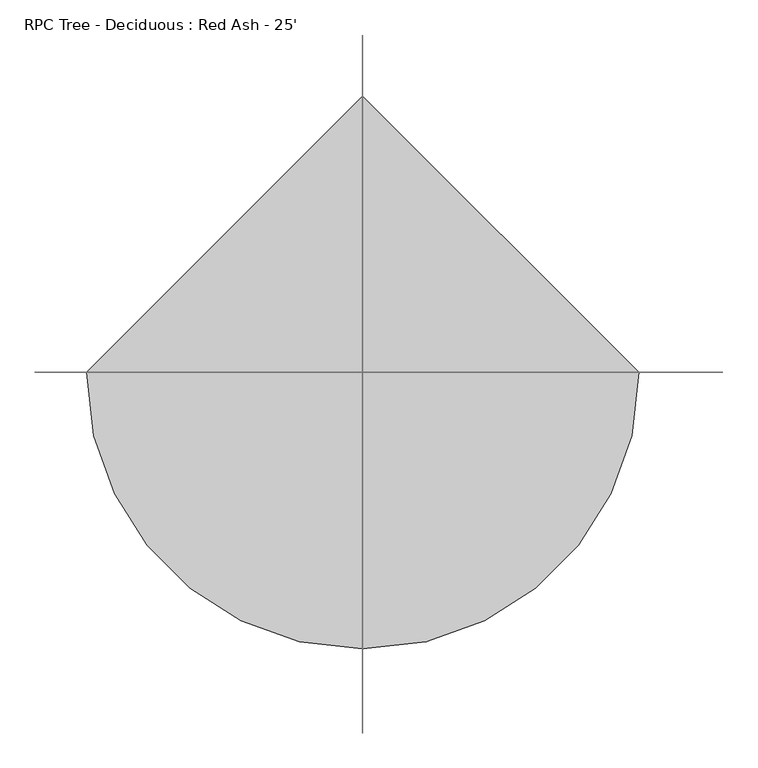
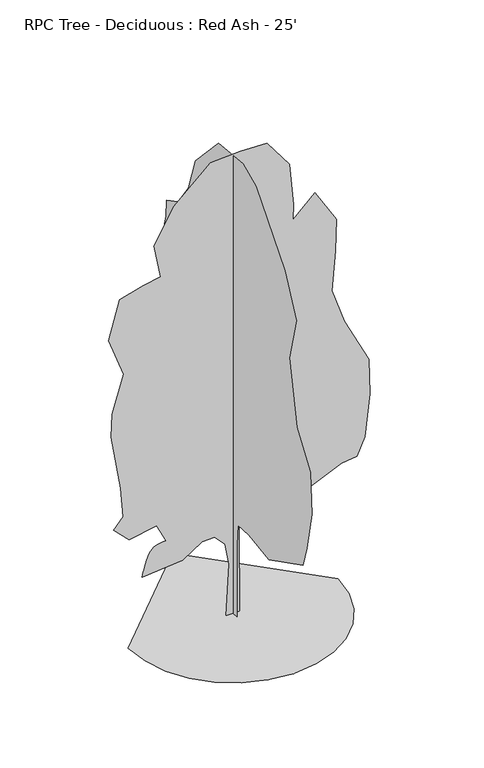
"""IFC4 building model written with IfcOpenShell, lengths in millimetres: geographic element geometry, RPC Tree - Deciduous : Red Ash - 25'."""

import ifcopenshell
import ifcopenshell.guid

model = None  # the IFC model being written
_history = None  # IfcOwnerHistory: only IFC2X3 demands one
_inside = {}  # id of a spatial element -> (the spatial element, [elements in it])
_under = {}  # id of a project, library or spatial element -> (it, [spatial elements below it])
_declared = {}  # id of a project -> (the project, [libraries it declares])
_typed = {}  # id of a type object -> (the type object, [elements of that type])
_made_of = {}  # id of a material, layer set ... -> (it, [elements and type objects made of it])


def new_model(schema):
    """Start an empty IFC model of exactly this schema.

    Asked for "IFC4X3", IfcOpenShell would pick the latest addendum, in which some entities
    have other attributes; the version numbers below select the first issue.
    IFC2X3 requires an IfcOwnerHistory on every rooted entity: one is made here for all.
    """
    global model, _history
    if schema == "IFC4X3":
        model = ifcopenshell.file(schema_version=(4, 3, 0, 0))
    else:
        model = ifcopenshell.file(schema=schema)
    _inside.clear()
    _under.clear()
    _declared.clear()
    _typed.clear()
    _made_of.clear()
    _history = None
    if model.schema == "IFC2X3":
        org = make("IfcOrganization", Name="unknown")
        user = make(
            "IfcPersonAndOrganization",
            ThePerson=make("IfcPerson", FamilyName="unknown"),
            TheOrganization=org,
        )
        app = make(
            "IfcApplication",
            ApplicationDeveloper=org,
            Version="unknown",
            ApplicationFullName="unknown",
            ApplicationIdentifier="unknown",
        )
        _history = make(
            "IfcOwnerHistory",
            OwningUser=user,
            OwningApplication=app,
            ChangeAction="ADDED",
            CreationDate=0,
        )
    return model


def make(cls, **values):
    """One entity of the class cls with the attributes given. An attribute that is None is left unset."""
    return model.create_entity(
        cls, **{name: value for name, value in values.items() if value is not None}
    )


def rooted(cls, **values):
    """An entity with a GlobalId (a new one), such as an element, a storey or a relation."""
    return make(cls, GlobalId=ifcopenshell.guid.new(), OwnerHistory=_history, **values)


def si_unit(unit_type, name, prefix=None):
    """IfcSIUnit, for example si_unit("LENGTHUNIT", "METRE", prefix="MILLI")."""
    return make("IfcSIUnit", UnitType=unit_type, Prefix=prefix, Name=name)


def assignment(units):
    """IfcUnitAssignment: the units of a project."""
    return None if units is None else make("IfcUnitAssignment", Units=units)


def point(xyz):
    """IfcCartesianPoint."""
    return None if xyz is None else make("IfcCartesianPoint", Coordinates=xyz)


def direction(xyz):
    """IfcDirection."""
    return None if xyz is None else make("IfcDirection", DirectionRatios=xyz)


def frame(location, z_axis=None, x_axis=None):
    """IfcAxis2Placement3D, a coordinate frame: its origin and axes. An axis left out is left unset."""
    return make(
        "IfcAxis2Placement3D",
        Location=point(location),
        Axis=direction(z_axis),
        RefDirection=direction(x_axis),
    )


def origin():
    """The frame at (0, 0, 0) with its axes left unset."""
    return frame((0.0, 0.0, 0.0))


def place(relative_to, where):
    """IfcLocalPlacement: puts the frame where relative to a parent placement (None: the world)."""
    return make(
        "IfcLocalPlacement", PlacementRelTo=relative_to, RelativePlacement=where
    )


def context(
    kind, dimensions, precision=None, world=None, true_north=None, identifier=None
):
    """IfcGeometricRepresentationContext, for example the 3D "Model" context."""
    return make(
        "IfcGeometricRepresentationContext",
        ContextIdentifier=identifier,
        ContextType=kind,
        CoordinateSpaceDimension=dimensions,
        Precision=precision,
        WorldCoordinateSystem=world,
        TrueNorth=true_north,
    )


def project(units=None, contexts=None):
    """IfcProject with its units and contexts."""
    return rooted(
        "IfcProject",
        Name="project",
        RepresentationContexts=contexts,
        UnitsInContext=assignment(units),
    )


def spatial(cls, under=None, at=None, **own):
    """A site, building, storey or space (cls), placed at a placement, below another one or the project."""
    s = rooted(cls, ObjectPlacement=at, **own)
    if under is not None:
        _under.setdefault(under.id(), (under, []))[1].append(s)
    return s


def point_list(points):
    """IfcCartesianPointList2D or 3D."""
    cls = (
        "IfcCartesianPointList2D" if len(points[0]) == 2 else "IfcCartesianPointList3D"
    )
    return make(cls, CoordList=points)


def triangles(points, corners, closed=None, point_numbers=None):
    """IfcTriangulatedFaceSet: each triangle names its three corners, points numbered from 1."""
    return make(
        "IfcTriangulatedFaceSet",
        Coordinates=point_list(points),
        Closed=closed,
        CoordIndex=corners,
        PnIndex=point_numbers,
    )


def shape(context_of_items, identifier, shape_type, items):
    """IfcShapeRepresentation: the items that make up one representation, for example the "Body"."""
    return make(
        "IfcShapeRepresentation",
        ContextOfItems=context_of_items,
        RepresentationIdentifier=identifier,
        RepresentationType=shape_type,
        Items=items,
    )


def source(mapping_origin, context_of_items, identifier, shape_type, items):
    """IfcRepresentationMap: a shape defined once, which mapped items show again and again."""
    return make(
        "IfcRepresentationMap",
        MappingOrigin=mapping_origin,
        MappedRepresentation=shape(context_of_items, identifier, shape_type, items),
    )


def transform(
    local_origin,
    x_axis=None,
    y_axis=None,
    z_axis=None,
    scale=None,
    scale2=None,
    scale3=None,
    uniform=True,
):
    """IfcCartesianTransformationOperator3D, or its non-uniform kind. x_axis, y_axis, z_axis: its Axis1, 2, 3."""
    if uniform:
        return make(
            "IfcCartesianTransformationOperator3D",
            Axis1=direction(x_axis),
            Axis2=direction(y_axis),
            LocalOrigin=point(local_origin),
            Scale=scale,
            Axis3=direction(z_axis),
        )
    return make(
        "IfcCartesianTransformationOperator3DnonUniform",
        Axis1=direction(x_axis),
        Axis2=direction(y_axis),
        LocalOrigin=point(local_origin),
        Scale=scale,
        Axis3=direction(z_axis),
        Scale2=scale2,
        Scale3=scale3,
    )


def mapped(mapping_source, mapping_target):
    """IfcMappedItem: shows the shape of a source again, moved by a transform."""
    return make(
        "IfcMappedItem", MappingSource=mapping_source, MappingTarget=mapping_target
    )


def made_of(thing, what):
    """Note that an element or type object is made of a material, layer set ...; save() writes the relation."""
    if what is not None:
        _made_of.setdefault(what.id(), (what, []))[1].append(thing)
    return thing


def element(
    cls,
    number,
    at=None,
    inside=None,
    cuts=None,
    type_object=None,
    material=None,
    context=None,
    identifier="Body",
    shape_type=None,
    held_by="IfcProductDefinitionShape",
    body=None,
    shapes=None,
    **own,
):
    """One element of the class cls, such as IfcWall. Its Tag is "e" and its number.

    at: its placement. inside: the storey or other place that contains it. cuts: it is an
    opening in that element (IfcRelVoidsElement). A single representation is given by context,
    identifier, shape_type and body (its items); several are given by shapes. held_by: the class
    of the entity that holds the representations. save() writes the other relations.
    """
    e = rooted(cls, Tag="e%d" % number, ObjectPlacement=at, **own)
    if body is not None:
        shapes = [shape(context, identifier, shape_type, body)]
    if shapes is not None:
        e.Representation = make(held_by, Representations=shapes)
    if inside is not None:
        _inside.setdefault(inside.id(), (inside, []))[1].append(e)
    if cuts is not None:
        rooted(
            "IfcRelVoidsElement", RelatingBuildingElement=cuts, RelatedOpeningElement=e
        )
    if type_object is not None:
        _typed.setdefault(type_object.id(), (type_object, []))[1].append(e)
    return made_of(e, material)


def aggregate(whole, parts):
    """IfcRelAggregates: a whole, such as a stair, and the parts it consists of."""
    return rooted("IfcRelAggregates", RelatingObject=whole, RelatedObjects=parts)


def save(model, path):
    """Write the relations noted so far, then the file.

    IfcRelAggregates (storeys below a building ...), IfcRelContainedInSpatialStructure (elements
    in a storey), IfcRelDefinesByType, IfcRelAssociatesMaterial and IfcRelDeclares: one each for
    every whole, place, type object, material and project.
    """
    for whole, parts in _under.values():
        aggregate(whole, parts)
    for where, things in _inside.values():
        rooted(
            "IfcRelContainedInSpatialStructure",
            RelatedElements=things,
            RelatingStructure=where,
        )
    for kind, things in _typed.values():
        rooted("IfcRelDefinesByType", RelatedObjects=things, RelatingType=kind)
    for what, things in _made_of.values():
        rooted("IfcRelAssociatesMaterial", RelatedObjects=things, RelatingMaterial=what)
    for by, libraries in _declared.values():
        rooted("IfcRelDeclares", RelatingContext=by, RelatedDefinitions=libraries)
    model.write(path)


def rpc_tree_deciduous_red_ash_25_14781bec(model_context):
    return source(origin(), model_context, "Body", "Tessellation", [
        triangles([(-1644.9525009, 0.0, 6.19e-05), (-1601.4651844, -376.9143482, 6.19e-05), (-1477.6144592, -723.0498339, 6.19e-05), (-1283.3164352, -1028.4894024, 6.19e-05), (-1028.4894751, -1283.3165806, 6.19e-05), (-723.0496885, -1477.6140232, 6.19e-05), (-376.9141665, -1601.4651844, 6.19e-05), (7.19e-05, -1644.9525009, 6.19e-05), (376.9143846, -1601.4651844, 6.19e-05), (723.0499065, -1477.6143139, 6.19e-05), (1028.4894751, -1283.3164352, 6.19e-05), (1283.3168713, -1028.4894751, 6.19e-05), (1477.6141685, -723.0496159, 6.19e-05), (1601.4651844, -376.9140939, 6.19e-05), (1644.9525009, 0.0001438, 6.19e-05), (-0.0002157, 1644.9525009, 6.19e-05), (-1.07e-05, -102.8462569, 0.0), (2.5e-05, -101.2467179, 1194.554048), (3.23e-05, -129.8819613, 1537.8029366), (7e-07, -438.8253948, 1558.1655018), (-5.78e-05, -976.3912743, 1478.3068588), (-0.0001405, -1903.692667, 1948.6771305), (-0.0001413, -2011.2060173, 2298.095192), (-0.0001361, -2145.5975235, 2943.1744217), (-0.0001119, -2105.2803623, 3615.1319527), (-5.81e-05, -1740.3819958, 4141.0172951), (-5.5e-06, -1527.3986298, 5160.6350006), (-3.5e-06, -1715.5451397, 5886.3488434), (4.79e-05, -1406.4449661, 6531.4286545), (0.0001569, -626.9743755, 7458.7301926), (0.0001985, -273.2007115, 7618.1942963), (0.0002662, 394.4016166, 7552.8046829), (0.0003121, 1026.0418774, 6880.8468613), (0.0003149, 1214.190204, 6316.4022446), (0.0003323, 1496.411277, 5913.2274353), (0.0003598, 1805.5131947, 5751.9582092), (0.0003531, 1818.9521999, 5483.1746155), (0.0003523, 1899.587249, 5174.0742966), (0.0003275, 1765.1957428, 4811.2170845), (0.0003297, 1886.1480984, 4461.7991684), (0.0003279, 2007.1004539, 3977.9897461), (0.0003211, 1980.222298, 3843.5979492), (0.0002877, 1751.7567375, 3521.0580437), (0.0002729, 1737.3115437, 3077.5662186), (0.0002632, 1724.8782909, 2795.3439102), (0.0002542, 1738.3174416, 2445.9262848), (0.0002412, 1751.7568829, 1962.1167171), (0.0002172, 1563.6084835, 1814.2857697), (0.0001807, 1214.1907127, 1814.2857697), (0.0001827, 1375.4605202, 1317.0371967), (0.0001715, 1348.4951603, 1034.8845062), (0.0001516, 1103.0310734, 1227.8363914), (9.86e-05, 629.4626684, 1106.7075932), (9.8e-05, 551.7118183, 1357.0609165), (6.29e-05, 215.9127657, 1354.0025276), (5.03e-05, 130.8012366, 1228.3346169), (3.27e-05, 79.5493323, 818.2831198), (1.17e-05, 112.1660096, 1.28e-05), (-110.870867, 4.8e-06, 4.46e-05), (-66.7114758, -9.64e-05, 833.5016676), (-129.3072962, -0.000136, 1187.9435503), (-290.7878647, -0.00015, 1365.31768), (-483.6364677, -0.0001408, 1358.6964272), (-796.2678211, -0.000103, 1155.7673166), (-1427.9080456, -6.9e-05, 1102.0108595), (-1419.1706429, -7.35e-05, 1136.7646975), (-1409.8454853, -7.82e-05, 1172.6938271), (-1399.3449635, -8.32e-05, 1210.9736853), (-1387.0813225, -8.87e-05, 1252.7803631), (-1372.4668076, -9.49e-05, 1299.2876987), (-1354.9136639, -0.0001019, 1351.6733093), (-1333.8341366, -0.0001099, 1411.1111057), (-1307.2693336, -0.0001176, 1466.2392815), (-1274.3570984, -0.0001239, 1506.556588), (-1236.1555058, -0.0001289, 1534.5316246), (-1193.7220493, -0.0001329, 1552.6338627), (-1148.1152401, -0.0001362, 1563.3300121), (-1100.3923536, -0.000139, 1569.0895443), (-1051.6116829, -0.0001415, 1572.3809132), (-1199.4421944, -0.0001703, 1868.0423721), (-1629.4953049, -0.0001418, 1787.4073231), (-1871.3997253, -0.0001601, 2029.3124702), (-1723.5690685, -0.0001874, 2204.0214283), (-1763.886375, -0.0002433, 2687.8309959), (-1911.7170319, -0.0003442, 3588.2539421), (-1898.4807758, -0.0003892, 3961.1654823), (-1719.9175472, -0.0004688, 4563.3255295), (-1952.0346291, -0.0005347, 5200.9523071), (-1777.3253803, -0.000616, 5819.1535263), (-1414.4687496, -0.0006447, 5926.6667313), (-1138.413216, -0.0006626, 5975.3625961), (-1239.7599369, -0.0007228, 6517.9893585), (-930.6591093, -0.000802, 7068.9952606), (-352.7753057, -0.0008898, 7593.1219894), (117.5946844, -0.0009135, 7620.0), (534.2087442, -0.0009301, 7606.5601227), (883.626733, -0.0008893, 7136.1905777), (947.8720848, -0.00081, 6447.5180786), (938.6469212, -0.0007795, 6194.9695404), (1286.8011063, -0.0008333, 6517.9893585), (1622.7800171, -0.0007823, 5966.9840378), (1609.3410118, -0.0007196, 5446.5094116), (1549.4574577, -0.00064, 4800.6520317), (1743.7323727, -0.0005809, 4233.3331718), (2131.7640656, -0.0005067, 3469.1978371), (2144.1354034, -0.0004386, 2892.8094727), (2066.2719875, -0.0003531, 2204.021283), (1945.319632, -0.0003141, 1921.7989746), (1703.4147755, -0.0003004, 1894.9206734), (1233.0446491, -0.0002542, 1679.8941181), (816.4305439, -0.0002007, 1384.2328045), (257.4765441, -0.0002049, 1624.5688614), (93.0508701, -0.0001766, 1447.6347485), (104.1552431, -4.6e-06, 3.52e-05)], [[15, 16, 1], [14, 15, 1], [14, 1, 2], [13, 14, 2], [13, 2, 3], [13, 3, 4], [12, 13, 4], [11, 12, 4], [11, 4, 5], [11, 5, 6], [11, 6, 7], [11, 7, 8], [11, 8, 9], [11, 9, 10], [50, 51, 52], [57, 58, 17], [57, 17, 18], [56, 57, 18], [56, 18, 19], [55, 56, 19], [49, 50, 52], [52, 53, 54], [49, 52, 54], [35, 36, 37], [46, 47, 48], [46, 48, 49], [21, 22, 23], [20, 21, 23], [20, 23, 24], [20, 24, 25], [20, 25, 26], [19, 20, 26], [19, 26, 27], [45, 46, 49], [31, 32, 33], [30, 31, 33], [29, 30, 33], [29, 33, 34], [28, 29, 34], [27, 28, 34], [19, 27, 34], [19, 34, 35], [19, 35, 37], [19, 37, 38], [19, 38, 39], [19, 39, 40], [19, 40, 41], [19, 41, 42], [19, 42, 43], [19, 43, 44], [19, 44, 45], [19, 45, 49], [19, 49, 54], [55, 19, 54], [64, 65, 66], [64, 66, 67], [64, 67, 68], [99, 100, 101], [64, 68, 69], [64, 69, 70], [64, 70, 71], [114, 59, 60], [113, 114, 60], [113, 60, 61], [113, 61, 62], [64, 71, 72], [64, 72, 73], [64, 73, 74], [64, 74, 75], [64, 75, 76], [64, 76, 77], [64, 77, 78], [64, 78, 79], [63, 64, 79], [81, 82, 83], [80, 81, 83], [99, 101, 102], [107, 108, 109], [110, 111, 112], [88, 89, 90], [87, 88, 90], [87, 90, 91], [80, 83, 84], [95, 96, 97], [95, 97, 98], [94, 95, 98], [93, 94, 98], [92, 93, 98], [91, 92, 98], [91, 98, 99], [87, 91, 99], [87, 99, 102], [87, 102, 103], [87, 103, 104], [86, 87, 104], [85, 86, 104], [84, 85, 104], [80, 84, 104], [80, 104, 105], [80, 105, 106], [80, 106, 107], [80, 107, 109], [80, 109, 110], [80, 110, 112], [79, 80, 112], [63, 79, 112], [62, 63, 112], [113, 62, 112]], closed=False),
    ])


if __name__ == "__main__":
    model = new_model("IFC4")
    model_context = context("Model", 3, world=origin())
    ifc_project = project(units=[si_unit("LENGTHUNIT", "METRE", prefix="MILLI")], contexts=[model_context])
    site = spatial("IfcSite", under=ifc_project)
    building = spatial("IfcBuilding", under=site)
    placement = place(None, origin())
    rpc_tree_deciduous_red_ash_25_shape = rpc_tree_deciduous_red_ash_25_14781bec(model_context)
    element("IfcGeographicElement", 1, ObjectType="RPC Tree - Deciduous : Red Ash - 25'", at=placement, inside=building, context=model_context, shape_type="MappedRepresentation", body=[
        mapped(rpc_tree_deciduous_red_ash_25_shape, transform((0.0, 0.0, 0.0), x_axis=(1.0, 0.0, 0.0), y_axis=(0.0, 1.0, 0.0), z_axis=(0.0, 0.0, 1.0))),
    ])
    save(model, "model.ifc")

# Revit data of these elements
# Type "RPC Tree - Deciduous : Red Ash - 25'"
#   COBie.Type.CreatedBy = "doug.wood@us.ibm.com"
#   COBie.Type.CreatedOn = "2016-04-14T02:07:24"
#   COBie.Type.Name = "Planting_RPC Tree - Deciduous_Red Ash - 25'"
#   COBie.Type.Category = "23-40 05 17 24 : Deciduous Trees"
#   COBie.Type.Description = "RPC Tree - Deciduous_Red Ash - 25'"
#   COBie.Type.Manufacturer = ""
#   COBie.Type.ModelNumber = ""
#   built-in parameter 1005198 = "{2, 15},{22, RPC-8-G3GR-497X-PHW5-6},{1, 0},{1, 0},{2, 15},{1, 8},{5, Color},{1, 0},{1, 0},{3, 0.8},{3, 0.8},{3, 0.8},{1, 8},{7, BBoxMin},{1, 0},{1, 0},{1, 0},{1, 0},{1, 0},{1, 8},{7, BBoxMax},{1, 0},{1, 0},{1, 0},{1, 0},{1, 0},{2, 11},{9, RPCTypeId},{1, 0},{1, 0},{22, RPC-8-G3GR-497X-PHW5-6},{1, 6},{14, RPCPlantHeight},{1, 0},{1, 0},{2, 25},{2, 11},{7, keyword},{1, 0},{1, 0},{34, :RPCs:Trees [General]:Geometry:RPC},{2, 11},{8, category},{1, 0},{1, 0},{15, Trees [General]},{2, 11},{12, LocalizedUID},{1, 0},{1, 0},{7, Red Ash},{2, 14},{6, Height},{1, 0},{1, 0},{2, 25},{1, 2},{16, Cast Reflections},{1, 0},{1, 0},{1, 0},{1, 2},{6, Jitter},{1, 0},{1, 0},{1, 1},{1, 2},{9, Billboard},{1, 0},{1, 0},{1, 0},{1, 2},{12, Cast Shadows},{1, 0},{1, 0},{1, 1},{1, 2},{20, Apply Filter Effects},{1, 0},{1, 0},{1, 0},{2, 11},{28, Apply Filter Effects-Text-FC},{1, 0},{1, 0},{4, None},{21, assetlibrary_base.fbx},{1, 5},"
#   built-in parameter 1005195 = "RPC-8-G3GR-497X-PHW5-6"
#   Type Comments = "Red Maple"
#   Assembly Code = "G2050500"
#   COBie.Type.ReplacementCost = 0
#   Height = 25' - 0"
#   COBie.Type = no
